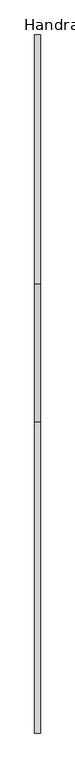
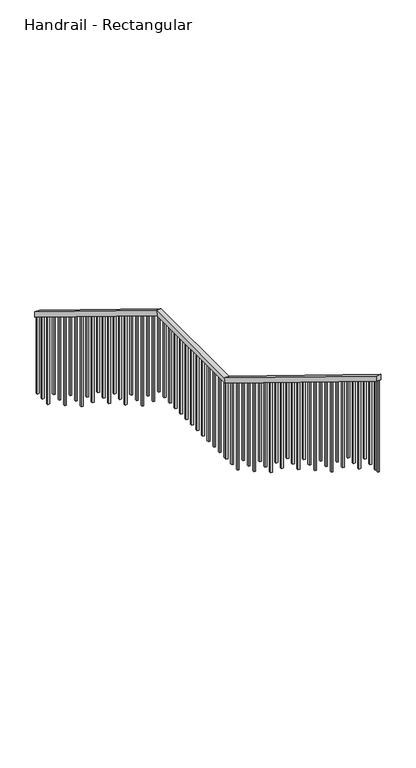
"""IFC4 building model written with IfcOpenShell, lengths in millimetres: railing geometry, Handrail - Rectangular."""

from ifc_helpers import new_model, si_unit, frame, origin, place, context, project, spatial, polyline, outline, extrude, faceted_brep, source, transform, mapped, element, save


def handrail_rectangular_a6e6b0f3(model_context):
    return source(origin(), model_context, "Body", "SolidModel", [
        faceted_brep([(476.2499995, 20358.1, 10452.1), (527.0499995, 20358.1, 10452.1), (527.0499995, 20358.1, 10392.4981634), (476.2499995, 20358.1, 10392.4981634), (476.2499995, 18122.9, 11823.7), (527.0499995, 18122.9, 11823.7), (527.0499995, 18108.5562663, 11772.9), (476.2499995, 18108.5562663, 11772.9), (476.2499995, 16878.3, 11823.7), (527.0499995, 16878.3, 11823.7), (527.0499995, 16863.9562663, 11772.9), (476.2499995, 16863.9562663, 11772.9), (476.2499995, 14084.3, 13538.2), (476.2499995, 14084.3, 13478.5981634), (527.0499995, 14084.3, 13478.5981634), (527.0499995, 14084.3, 13538.2)], [[[0, 1, 2, 3]], [[1, 0, 4, 5]], [[2, 1, 5, 6]], [[3, 2, 6, 7]], [[0, 3, 7, 4]], [[5, 4, 8, 9]], [[6, 5, 9, 10]], [[7, 6, 10, 11]], [[4, 7, 11, 8]], [[12, 13, 14, 15]], [[9, 8, 12, 15]], [[10, 9, 15, 14]], [[11, 10, 14, 13]], [[8, 11, 13, 12]]]),
        extrude(outline(polyline([(14125.575, 13453.2703225), (14144.625, 13441.5805498), (14144.625, 12452.35), (14125.575, 12452.35), (14125.575, 13453.2703225)])), frame((492.1249995, 0.0, 0.0), z_axis=(1.0, 0.0, 0.0), x_axis=(0.0, 1.0, 0.0)), (0.0, 0.0, 1.0), 19.05),
        extrude(outline(polyline([(14227.175, 13390.9248679), (14246.225, 13379.2350952), (14246.225, 12452.35), (14227.175, 12452.35), (14227.175, 13390.9248679)])), frame((492.1249995, 0.0, 0.0), z_axis=(1.0, 0.0, 0.0), x_axis=(0.0, 1.0, 0.0)), (0.0, 0.0, 1.0), 19.05),
        extrude(outline(polyline([(14328.775, 13328.5794134), (14347.825, 13316.8896407), (14347.825, 12452.35), (14328.775, 12452.35), (14328.775, 13328.5794134)])), frame((492.1249995, 0.0, 0.0), z_axis=(1.0, 0.0, 0.0), x_axis=(0.0, 1.0, 0.0)), (0.0, 0.0, 1.0), 19.05),
        extrude(outline(polyline([(14430.375, 13266.2339589), (14449.425, 13254.5441861), (14449.425, 12280.9), (14430.375, 12280.9), (14430.375, 13266.2339589)])), frame((492.1249995, 0.0, 0.0), z_axis=(1.0, 0.0, 0.0), x_axis=(0.0, 1.0, 0.0)), (0.0, 0.0, 1.0), 19.05),
        extrude(outline(polyline([(14531.975, 13203.8885043), (14551.025, 13192.1987316), (14551.025, 12280.9), (14531.975, 12280.9), (14531.975, 13203.8885043)])), frame((492.1249995, 0.0, 0.0), z_axis=(1.0, 0.0, 0.0), x_axis=(0.0, 1.0, 0.0)), (0.0, 0.0, 1.0), 19.05),
        extrude(outline(polyline([(14633.575, 13141.5430498), (14652.625, 13129.853277), (14652.625, 12280.9), (14633.575, 12280.9), (14633.575, 13141.5430498)])), frame((492.1249995, 0.0, 0.0), z_axis=(1.0, 0.0, 0.0), x_axis=(0.0, 1.0, 0.0)), (0.0, 0.0, 1.0), 19.05),
        extrude(outline(polyline([(14735.175, 13079.1975952), (14754.225, 13067.5078225), (14754.225, 12109.45), (14735.175, 12109.45), (14735.175, 13079.1975952)])), frame((492.1249995, 0.0, 0.0), z_axis=(1.0, 0.0, 0.0), x_axis=(0.0, 1.0, 0.0)), (0.0, 0.0, 1.0), 19.05),
        extrude(outline(polyline([(14836.775, 13016.8521407), (14855.825, 13005.1623679), (14855.825, 12109.45), (14836.775, 12109.45), (14836.775, 13016.8521407)])), frame((492.1249995, 0.0, 0.0), z_axis=(1.0, 0.0, 0.0), x_axis=(0.0, 1.0, 0.0)), (0.0, 0.0, 1.0), 19.05),
        extrude(outline(polyline([(14938.375, 12954.5066861), (14957.425, 12942.8169134), (14957.425, 11938.0), (14938.375, 11938.0), (14938.375, 12954.5066861)])), frame((492.1249995, 0.0, 0.0), z_axis=(1.0, 0.0, 0.0), x_axis=(0.0, 1.0, 0.0)), (0.0, 0.0, 1.0), 19.05),
        extrude(outline(polyline([(15039.975, 12892.1612316), (15059.025, 12880.4714589), (15059.025, 11938.0), (15039.975, 11938.0), (15039.975, 12892.1612316)])), frame((492.1249995, 0.0, 0.0), z_axis=(1.0, 0.0, 0.0), x_axis=(0.0, 1.0, 0.0)), (0.0, 0.0, 1.0), 19.05),
        extrude(outline(polyline([(15141.575, 12829.815777), (15160.625, 12818.1260043), (15160.625, 11938.0), (15141.575, 11938.0), (15141.575, 12829.815777)])), frame((492.1249995, 0.0, 0.0), z_axis=(1.0, 0.0, 0.0), x_axis=(0.0, 1.0, 0.0)), (0.0, 0.0, 1.0), 19.05),
        extrude(outline(polyline([(15243.175, 12767.4703225), (15262.225, 12755.7805498), (15262.225, 11766.55), (15243.175, 11766.55), (15243.175, 12767.4703225)])), frame((492.1249995, 0.0, 0.0), z_axis=(1.0, 0.0, 0.0), x_axis=(0.0, 1.0, 0.0)), (0.0, 0.0, 1.0), 19.05),
        extrude(outline(polyline([(15344.775, 12705.1248679), (15363.825, 12693.4350952), (15363.825, 11766.55), (15344.775, 11766.55), (15344.775, 12705.1248679)])), frame((492.1249995, 0.0, 0.0), z_axis=(1.0, 0.0, 0.0), x_axis=(0.0, 1.0, 0.0)), (0.0, 0.0, 1.0), 19.05),
        extrude(outline(polyline([(15446.375, 12642.7794134), (15465.425, 12631.0896407), (15465.425, 11766.55), (15446.375, 11766.55), (15446.375, 12642.7794134)])), frame((492.1249995, 0.0, 0.0), z_axis=(1.0, 0.0, 0.0), x_axis=(0.0, 1.0, 0.0)), (0.0, 0.0, 1.0), 19.05),
        extrude(outline(polyline([(15547.975, 12580.4339589), (15567.025, 12568.7441861), (15567.025, 11595.1), (15547.975, 11595.1), (15547.975, 12580.4339589)])), frame((492.1249995, 0.0, 0.0), z_axis=(1.0, 0.0, 0.0), x_axis=(0.0, 1.0, 0.0)), (0.0, 0.0, 1.0), 19.05),
        extrude(outline(polyline([(15649.575, 12518.0885043), (15668.625, 12506.3987316), (15668.625, 11595.1), (15649.575, 11595.1), (15649.575, 12518.0885043)])), frame((492.1249995, 0.0, 0.0), z_axis=(1.0, 0.0, 0.0), x_axis=(0.0, 1.0, 0.0)), (0.0, 0.0, 1.0), 19.05),
        extrude(outline(polyline([(15751.175, 12455.7430498), (15770.225, 12444.053277), (15770.225, 11595.1), (15751.175, 11595.1), (15751.175, 12455.7430498)])), frame((492.1249995, 0.0, 0.0), z_axis=(1.0, 0.0, 0.0), x_axis=(0.0, 1.0, 0.0)), (0.0, 0.0, 1.0), 19.05),
        extrude(outline(polyline([(15852.775, 12393.3975952), (15871.825, 12381.7078225), (15871.825, 11423.65), (15852.775, 11423.65), (15852.775, 12393.3975952)])), frame((492.1249995, 0.0, 0.0), z_axis=(1.0, 0.0, 0.0), x_axis=(0.0, 1.0, 0.0)), (0.0, 0.0, 1.0), 19.05),
        extrude(outline(polyline([(15954.375, 12331.0521407), (15973.425, 12319.3623679), (15973.425, 11423.65), (15954.375, 11423.65), (15954.375, 12331.0521407)])), frame((492.1249995, 0.0, 0.0), z_axis=(1.0, 0.0, 0.0), x_axis=(0.0, 1.0, 0.0)), (0.0, 0.0, 1.0), 19.05),
        extrude(outline(polyline([(16055.975, 12268.7066861), (16075.025, 12257.0169134), (16075.025, 11252.2), (16055.975, 11252.2), (16055.975, 12268.7066861)])), frame((492.1249995, 0.0, 0.0), z_axis=(1.0, 0.0, 0.0), x_axis=(0.0, 1.0, 0.0)), (0.0, 0.0, 1.0), 19.05),
        extrude(outline(polyline([(16157.575, 12206.3612316), (16176.625, 12194.6714589), (16176.625, 11252.2), (16157.575, 11252.2), (16157.575, 12206.3612316)])), frame((492.1249995, 0.0, 0.0), z_axis=(1.0, 0.0, 0.0), x_axis=(0.0, 1.0, 0.0)), (0.0, 0.0, 1.0), 19.05),
        extrude(outline(polyline([(16259.175, 12144.015777), (16278.225, 12132.3260043), (16278.225, 11252.2), (16259.175, 11252.2), (16259.175, 12144.015777)])), frame((492.1249995, 0.0, 0.0), z_axis=(1.0, 0.0, 0.0), x_axis=(0.0, 1.0, 0.0)), (0.0, 0.0, 1.0), 19.05),
        extrude(outline(polyline([(16360.775, 12081.6703225), (16379.825, 12069.9805498), (16379.825, 11080.75), (16360.775, 11080.75), (16360.775, 12081.6703225)])), frame((492.1249995, 0.0, 0.0), z_axis=(1.0, 0.0, 0.0), x_axis=(0.0, 1.0, 0.0)), (0.0, 0.0, 1.0), 19.05),
        extrude(outline(polyline([(16462.375, 12019.3248679), (16481.425, 12007.6350952), (16481.425, 11080.75), (16462.375, 11080.75), (16462.375, 12019.3248679)])), frame((492.1249995, 0.0, 0.0), z_axis=(1.0, 0.0, 0.0), x_axis=(0.0, 1.0, 0.0)), (0.0, 0.0, 1.0), 19.05),
        extrude(outline(polyline([(16563.975, 11956.9794134), (16583.025, 11945.2896407), (16583.025, 11080.75), (16563.975, 11080.75), (16563.975, 11956.9794134)])), frame((492.1249995, 0.0, 0.0), z_axis=(1.0, 0.0, 0.0), x_axis=(0.0, 1.0, 0.0)), (0.0, 0.0, 1.0), 19.05),
        extrude(outline(polyline([(16665.575, 11894.6339589), (16684.625, 11882.9441861), (16684.625, 10909.3), (16665.575, 10909.3), (16665.575, 11894.6339589)])), frame((492.1249995, 0.0, 0.0), z_axis=(1.0, 0.0, 0.0), x_axis=(0.0, 1.0, 0.0)), (0.0, 0.0, 1.0), 19.05),
        extrude(outline(polyline([(16767.175, 11832.2885043), (16786.225, 11820.5987316), (16786.225, 10909.3), (16767.175, 10909.3), (16767.175, 11832.2885043)])), frame((492.1249995, 0.0, 0.0), z_axis=(1.0, 0.0, 0.0), x_axis=(0.0, 1.0, 0.0)), (0.0, 0.0, 1.0), 19.05),
        extrude(outline(polyline([(492.1249995, 16913.225), (511.1749995, 16913.225), (511.1749995, 16894.175), (492.1249995, 16894.175), (492.1249995, 16913.225)])), frame((0.0, 0.0, 10909.3), z_axis=(0.0, 0.0, 1.0), x_axis=(1.0, 0.0, 0.0)), (0.0, 0.0, 1.0), 863.6),
        extrude(outline(polyline([(492.1249995, 17014.825), (511.1749995, 17014.825), (511.1749995, 16995.775), (492.1249995, 16995.775), (492.1249995, 17014.825)])), frame((0.0, 0.0, 10909.3), z_axis=(0.0, 0.0, 1.0), x_axis=(1.0, 0.0, 0.0)), (0.0, 0.0, 1.0), 863.6),
        extrude(outline(polyline([(492.1249995, 17116.425), (511.1749995, 17116.425), (511.1749995, 17097.375), (492.1249995, 17097.375), (492.1249995, 17116.425)])), frame((0.0, 0.0, 10909.3), z_axis=(0.0, 0.0, 1.0), x_axis=(1.0, 0.0, 0.0)), (0.0, 0.0, 1.0), 863.6),
        extrude(outline(polyline([(492.1249995, 17218.025), (511.1749995, 17218.025), (511.1749995, 17198.975), (492.1249995, 17198.975), (492.1249995, 17218.025)])), frame((0.0, 0.0, 10909.3), z_axis=(0.0, 0.0, 1.0), x_axis=(1.0, 0.0, 0.0)), (0.0, 0.0, 1.0), 863.6),
        extrude(outline(polyline([(492.1249995, 17319.625), (511.1749995, 17319.625), (511.1749995, 17300.575), (492.1249995, 17300.575), (492.1249995, 17319.625)])), frame((0.0, 0.0, 10909.3), z_axis=(0.0, 0.0, 1.0), x_axis=(1.0, 0.0, 0.0)), (0.0, 0.0, 1.0), 863.6),
        extrude(outline(polyline([(492.1249995, 17421.225), (511.1749995, 17421.225), (511.1749995, 17402.175), (492.1249995, 17402.175), (492.1249995, 17421.225)])), frame((0.0, 0.0, 10909.3), z_axis=(0.0, 0.0, 1.0), x_axis=(1.0, 0.0, 0.0)), (0.0, 0.0, 1.0), 863.6),
        extrude(outline(polyline([(492.1249995, 17522.825), (511.1749995, 17522.825), (511.1749995, 17503.775), (492.1249995, 17503.775), (492.1249995, 17522.825)])), frame((0.0, 0.0, 10909.3), z_axis=(0.0, 0.0, 1.0), x_axis=(1.0, 0.0, 0.0)), (0.0, 0.0, 1.0), 863.6),
        extrude(outline(polyline([(492.1249995, 17624.425), (511.1749995, 17624.425), (511.1749995, 17605.375), (492.1249995, 17605.375), (492.1249995, 17624.425)])), frame((0.0, 0.0, 10909.3), z_axis=(0.0, 0.0, 1.0), x_axis=(1.0, 0.0, 0.0)), (0.0, 0.0, 1.0), 863.6),
        extrude(outline(polyline([(492.1249995, 17726.025), (511.1749995, 17726.025), (511.1749995, 17706.975), (492.1249995, 17706.975), (492.1249995, 17726.025)])), frame((0.0, 0.0, 10909.3), z_axis=(0.0, 0.0, 1.0), x_axis=(1.0, 0.0, 0.0)), (0.0, 0.0, 1.0), 863.6),
        extrude(outline(polyline([(492.1249995, 17827.625), (511.1749995, 17827.625), (511.1749995, 17808.575), (492.1249995, 17808.575), (492.1249995, 17827.625)])), frame((0.0, 0.0, 10909.3), z_axis=(0.0, 0.0, 1.0), x_axis=(1.0, 0.0, 0.0)), (0.0, 0.0, 1.0), 863.6),
        extrude(outline(polyline([(492.1249995, 17929.225), (511.1749995, 17929.225), (511.1749995, 17910.175), (492.1249995, 17910.175), (492.1249995, 17929.225)])), frame((0.0, 0.0, 10909.3), z_axis=(0.0, 0.0, 1.0), x_axis=(1.0, 0.0, 0.0)), (0.0, 0.0, 1.0), 863.6),
        extrude(outline(polyline([(492.1249995, 18030.825), (511.1749995, 18030.825), (511.1749995, 18011.775), (492.1249995, 18011.775), (492.1249995, 18030.825)])), frame((0.0, 0.0, 10909.3), z_axis=(0.0, 0.0, 1.0), x_axis=(1.0, 0.0, 0.0)), (0.0, 0.0, 1.0), 863.6),
        extrude(outline(polyline([(18214.975, 11707.5975952), (18234.025, 11695.9078225), (18234.025, 10737.85), (18214.975, 10737.85), (18214.975, 11707.5975952)])), frame((492.1249995, 0.0, 0.0), z_axis=(1.0, 0.0, 0.0), x_axis=(0.0, 1.0, 0.0)), (0.0, 0.0, 1.0), 19.05),
        extrude(outline(polyline([(18316.575, 11645.2521407), (18335.625, 11633.5623679), (18335.625, 10737.85), (18316.575, 10737.85), (18316.575, 11645.2521407)])), frame((492.1249995, 0.0, 0.0), z_axis=(1.0, 0.0, 0.0), x_axis=(0.0, 1.0, 0.0)), (0.0, 0.0, 1.0), 19.05),
        extrude(outline(polyline([(18418.175, 11582.9066861), (18437.225, 11571.2169134), (18437.225, 10566.4), (18418.175, 10566.4), (18418.175, 11582.9066861)])), frame((492.1249995, 0.0, 0.0), z_axis=(1.0, 0.0, 0.0), x_axis=(0.0, 1.0, 0.0)), (0.0, 0.0, 1.0), 19.05),
        extrude(outline(polyline([(18519.775, 11520.5612316), (18538.825, 11508.8714589), (18538.825, 10566.4), (18519.775, 10566.4), (18519.775, 11520.5612316)])), frame((492.1249995, 0.0, 0.0), z_axis=(1.0, 0.0, 0.0), x_axis=(0.0, 1.0, 0.0)), (0.0, 0.0, 1.0), 19.05),
        extrude(outline(polyline([(18621.375, 11458.215777), (18640.425, 11446.5260043), (18640.425, 10566.4), (18621.375, 10566.4), (18621.375, 11458.215777)])), frame((492.1249995, 0.0, 0.0), z_axis=(1.0, 0.0, 0.0), x_axis=(0.0, 1.0, 0.0)), (0.0, 0.0, 1.0), 19.05),
        extrude(outline(polyline([(18722.975, 11395.8703225), (18742.025, 11384.1805498), (18742.025, 10394.95), (18722.975, 10394.95), (18722.975, 11395.8703225)])), frame((492.1249995, 0.0, 0.0), z_axis=(1.0, 0.0, 0.0), x_axis=(0.0, 1.0, 0.0)), (0.0, 0.0, 1.0), 19.05),
        extrude(outline(polyline([(18824.575, 11333.5248679), (18843.625, 11321.8350952), (18843.625, 10394.95), (18824.575, 10394.95), (18824.575, 11333.5248679)])), frame((492.1249995, 0.0, 0.0), z_axis=(1.0, 0.0, 0.0), x_axis=(0.0, 1.0, 0.0)), (0.0, 0.0, 1.0), 19.05),
        extrude(outline(polyline([(18926.175, 11271.1794134), (18945.225, 11259.4896407), (18945.225, 10394.95), (18926.175, 10394.95), (18926.175, 11271.1794134)])), frame((492.1249995, 0.0, 0.0), z_axis=(1.0, 0.0, 0.0), x_axis=(0.0, 1.0, 0.0)), (0.0, 0.0, 1.0), 19.05),
        extrude(outline(polyline([(19027.775, 11208.8339589), (19046.825, 11197.1441861), (19046.825, 10223.5), (19027.775, 10223.5), (19027.775, 11208.8339589)])), frame((492.1249995, 0.0, 0.0), z_axis=(1.0, 0.0, 0.0), x_axis=(0.0, 1.0, 0.0)), (0.0, 0.0, 1.0), 19.05),
        extrude(outline(polyline([(19129.375, 11146.4885043), (19148.425, 11134.7987316), (19148.425, 10223.5), (19129.375, 10223.5), (19129.375, 11146.4885043)])), frame((492.1249995, 0.0, 0.0), z_axis=(1.0, 0.0, 0.0), x_axis=(0.0, 1.0, 0.0)), (0.0, 0.0, 1.0), 19.05),
        extrude(outline(polyline([(19230.975, 11084.1430498), (19250.025, 11072.453277), (19250.025, 10223.5), (19230.975, 10223.5), (19230.975, 11084.1430498)])), frame((492.1249995, 0.0, 0.0), z_axis=(1.0, 0.0, 0.0), x_axis=(0.0, 1.0, 0.0)), (0.0, 0.0, 1.0), 19.05),
        extrude(outline(polyline([(19332.575, 11021.7975952), (19351.625, 11010.1078225), (19351.625, 10052.05), (19332.575, 10052.05), (19332.575, 11021.7975952)])), frame((492.1249995, 0.0, 0.0), z_axis=(1.0, 0.0, 0.0), x_axis=(0.0, 1.0, 0.0)), (0.0, 0.0, 1.0), 19.05),
        extrude(outline(polyline([(19434.175, 10959.4521407), (19453.225, 10947.7623679), (19453.225, 10052.05), (19434.175, 10052.05), (19434.175, 10959.4521407)])), frame((492.1249995, 0.0, 0.0), z_axis=(1.0, 0.0, 0.0), x_axis=(0.0, 1.0, 0.0)), (0.0, 0.0, 1.0), 19.05),
        extrude(outline(polyline([(19535.775, 10897.1066861), (19554.825, 10885.4169134), (19554.825, 9880.6), (19535.775, 9880.6), (19535.775, 10897.1066861)])), frame((492.1249995, 0.0, 0.0), z_axis=(1.0, 0.0, 0.0), x_axis=(0.0, 1.0, 0.0)), (0.0, 0.0, 1.0), 19.05),
        extrude(outline(polyline([(19637.375, 10834.7612316), (19656.425, 10823.0714589), (19656.425, 9880.6), (19637.375, 9880.6), (19637.375, 10834.7612316)])), frame((492.1249995, 0.0, 0.0), z_axis=(1.0, 0.0, 0.0), x_axis=(0.0, 1.0, 0.0)), (0.0, 0.0, 1.0), 19.05),
        extrude(outline(polyline([(19738.975, 10772.415777), (19758.025, 10760.7260043), (19758.025, 9880.6), (19738.975, 9880.6), (19738.975, 10772.415777)])), frame((492.1249995, 0.0, 0.0), z_axis=(1.0, 0.0, 0.0), x_axis=(0.0, 1.0, 0.0)), (0.0, 0.0, 1.0), 19.05),
        extrude(outline(polyline([(19840.575, 10710.0703225), (19859.625, 10698.3805498), (19859.625, 9709.15), (19840.575, 9709.15), (19840.575, 10710.0703225)])), frame((492.1249995, 0.0, 0.0), z_axis=(1.0, 0.0, 0.0), x_axis=(0.0, 1.0, 0.0)), (0.0, 0.0, 1.0), 19.05),
        extrude(outline(polyline([(19942.175, 10647.7248679), (19961.225, 10636.0350952), (19961.225, 9709.15), (19942.175, 9709.15), (19942.175, 10647.7248679)])), frame((492.1249995, 0.0, 0.0), z_axis=(1.0, 0.0, 0.0), x_axis=(0.0, 1.0, 0.0)), (0.0, 0.0, 1.0), 19.05),
        extrude(outline(polyline([(20043.775, 10585.3794134), (20062.825, 10573.6896407), (20062.825, 9709.15), (20043.775, 9709.15), (20043.775, 10585.3794134)])), frame((492.1249995, 0.0, 0.0), z_axis=(1.0, 0.0, 0.0), x_axis=(0.0, 1.0, 0.0)), (0.0, 0.0, 1.0), 19.05),
        extrude(outline(polyline([(20145.375, 10523.0339589), (20164.425, 10511.3441861), (20164.425, 9537.7), (20145.375, 9537.7), (20145.375, 10523.0339589)])), frame((492.1249995, 0.0, 0.0), z_axis=(1.0, 0.0, 0.0), x_axis=(0.0, 1.0, 0.0)), (0.0, 0.0, 1.0), 19.05),
        extrude(outline(polyline([(20246.975, 10460.6885043), (20266.025, 10448.9987316), (20266.025, 9537.7), (20246.975, 9537.7), (20246.975, 10460.6885043)])), frame((492.1249995, 0.0, 0.0), z_axis=(1.0, 0.0, 0.0), x_axis=(0.0, 1.0, 0.0)), (0.0, 0.0, 1.0), 19.05),
        extrude(outline(polyline([(492.1249995, 16887.825), (511.1749995, 16887.825), (511.1749995, 16868.775), (492.1249995, 16868.775), (492.1249995, 16887.825)])), frame((0.0, 0.0, 10909.3), z_axis=(0.0, 0.0, 1.0), x_axis=(1.0, 0.0, 0.0)), (0.0, 0.0, 1.0), 863.6),
        extrude(outline(polyline([(18113.375, 11769.9430498), (18132.425, 11758.253277), (18132.425, 10909.3), (18113.375, 10909.3), (18113.375, 11769.9430498)])), frame((492.1249995, 0.0, 0.0), z_axis=(1.0, 0.0, 0.0), x_axis=(0.0, 1.0, 0.0)), (0.0, 0.0, 1.0), 19.05),
        extrude(outline(polyline([(14084.3, 13478.5981634), (14103.35, 13466.9083907), (14103.35, 12452.35), (14084.3, 12452.35), (14084.3, 13478.5981634)])), frame((492.1249995, 0.0, 0.0), z_axis=(1.0, 0.0, 0.0), x_axis=(0.0, 1.0, 0.0)), (0.0, 0.0, 1.0), 19.05),
        extrude(outline(polyline([(20339.05, 10404.1879361), (20358.1, 10392.4981634), (20358.1, 9537.7), (20339.05, 9537.7), (20339.05, 10404.1879361)])), frame((492.1249995, 0.0, 0.0), z_axis=(1.0, 0.0, 0.0), x_axis=(0.0, 1.0, 0.0)), (0.0, 0.0, 1.0), 19.05),
    ])


if __name__ == "__main__":
    model = new_model("IFC4")
    model_context = context("Model", 3, world=origin())
    ifc_project = project(units=[si_unit("LENGTHUNIT", "METRE", prefix="MILLI")], contexts=[model_context])
    site = spatial("IfcSite", under=ifc_project)
    building = spatial("IfcBuilding", under=site)
    placement = place(None, origin())
    handrail_rectangular_shape = handrail_rectangular_a6e6b0f3(model_context)
    element("IfcRailing", 1, ObjectType="Handrail - Rectangular", at=placement, inside=building, context=model_context, shape_type="MappedRepresentation", body=[
        mapped(handrail_rectangular_shape, transform((0.0, 0.0, 0.0), x_axis=(1.0, 0.0, 0.0), y_axis=(0.0, 1.0, 0.0), z_axis=(0.0, 0.0, 1.0))),
    ])
    save(model, "model.ifc")
